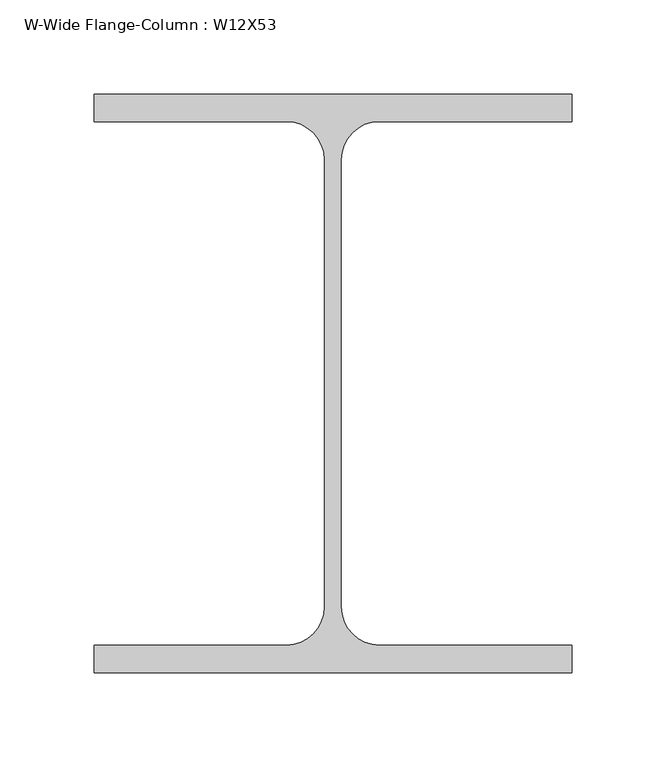
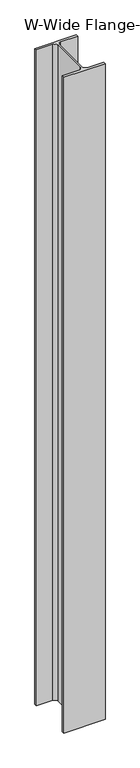
"""IFC4 building model written with IfcOpenShell, lengths in millimetres: column geometry, W-Wide Flange-Column : W12X53."""

from ifc_helpers import new_model, si_unit, point, frame, frame_2d, origin, place, context, project, spatial, polyline, circle_curve, trimmed, segment, composite_curve, outline, extrude, source, transform, mapped, element, save


def w_wide_flange_column_w12x53_00415955(model_context):
    return source(origin(), model_context, "Body", "SweptSolid", [
        extrude(outline(composite_curve([segment(polyline([(127.0, 153.67), (127.0, 139.065), (24.7015, 139.065)]), True, "CONTINUOUS"), segment(trimmed(circle_curve(frame_2d((24.7015, 118.745)), 20.32), [point((24.7015, 139.065))], [point((4.3815, 118.745))], True, "CARTESIAN"), True, "CONTINUOUS"), segment(polyline([(4.3815, 118.745), (4.3815, -118.745)]), True, "CONTINUOUS"), segment(trimmed(circle_curve(frame_2d((24.7015, -118.745)), 20.32), [point((4.3815, -118.745))], [point((24.7015, -139.065))], True, "CARTESIAN"), True, "CONTINUOUS"), segment(polyline([(24.7015, -139.065), (127.0, -139.065), (127.0, -153.67), (-127.0, -153.67), (-127.0, -139.065), (-24.7015, -139.065)]), True, "CONTINUOUS"), segment(trimmed(circle_curve(frame_2d((-24.7015, -118.745)), 20.32), [point((-24.7015, -139.065))], [point((-4.3815, -118.745))], True, "CARTESIAN"), True, "CONTINUOUS"), segment(polyline([(-4.3815, -118.745), (-4.3815, 118.745)]), True, "CONTINUOUS"), segment(trimmed(circle_curve(frame_2d((-24.7015, 118.745)), 20.32), [point((-4.3815, 118.745))], [point((-24.7015, 139.065))], True, "CARTESIAN"), True, "CONTINUOUS"), segment(polyline([(-24.7015, 139.065), (-127.0, 139.065), (-127.0, 153.67), (127.0, 153.67)]), True, "CONTINUOUS")], self_intersect=False)), frame((0.0, 0.0, 23317.2), z_axis=(0.0, 0.0, 1.0), x_axis=(1.0, 0.0, 0.0)), (0.0, 0.0, 1.0), 4267.2),
    ])


if __name__ == "__main__":
    model = new_model("IFC4")
    model_context = context("Model", 3, world=origin())
    ifc_project = project(units=[si_unit("LENGTHUNIT", "METRE", prefix="MILLI")], contexts=[model_context])
    site = spatial("IfcSite", under=ifc_project)
    building = spatial("IfcBuilding", under=site)
    placement = place(None, origin())
    w_wide_flange_column_w12x53_shape = w_wide_flange_column_w12x53_00415955(model_context)
    element("IfcColumn", 1, ObjectType="W-Wide Flange-Column : W12X53", at=placement, inside=building, context=model_context, shape_type="MappedRepresentation", body=[
        mapped(w_wide_flange_column_w12x53_shape, transform((0.0, 0.0, 0.0), x_axis=(1.0, 0.0, 0.0), y_axis=(0.0, 1.0, 0.0), z_axis=(0.0, 0.0, 1.0))),
    ])
    save(model, "model.ifc")

# Revit data of these elements
# Project information
#   TBC Electrician = "ELECTRICIAN HERE"
#   TBC Fire Protection = "FP HERE"
#   TBC Plumber = "PLUMBER HERE"
#   TBC HVAC = "HVAC HERE"
#   TBC Other Company 1 = "MISC COMPANY 1"
#   TBC Other Company 2 = "MISC COMPANY 2"
#   TBC COORDINATOR = "NAME OF VCC"
#   Project Issue Date = "2010.12.07"
#   Project Status = "Project Status"
#   Client Name = "Owner"
#   Project Address = "111 BOYLSTON STREET, \nBROOKLINE MA"
#   Project Name = "HOMEWOOD SUITES"
#   Project Number = "13381"
# Type "W-Wide Flange-Column : W12X53"
#   Assembly Code = "B10"
#   W = 53
#   bf = 0' - 10"
#   d = 1' - 0.1"
#   k = 0' - 1 3/8"
#   kr = 0' - 0.8"
#   tf = 0' - 0.575"
#   tw = 0' - 0.345"
#   A = 0.108333 SF
#   Structural Material [instance default] = Steel ASTM A992
# Element 1 (IfcColumn, "W-Wide Flange-Column : W12X53")
#   Materials on its faces: "Steel ASTM A992"
# Materials
#   "Steel ASTM A992": class "Metal", colour RGB 199 199 199, transparency 0, Description = "Structural steel 50ksi", Cost = 0
